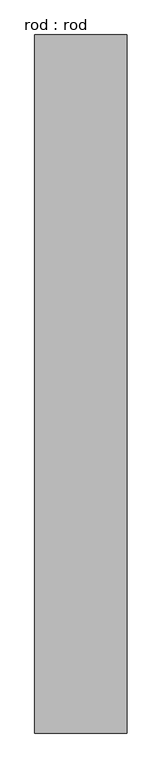
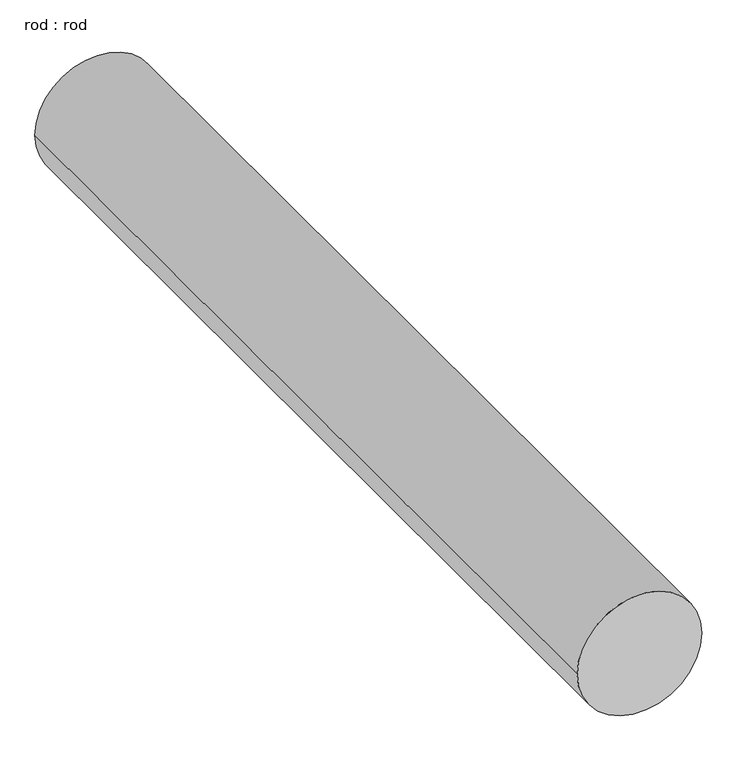
"""IFC4 building model written with IfcOpenShell, lengths in millimetres: proxy geometry, rod : rod."""

from ifc_helpers import new_model, si_unit, point, frame, frame_2d, origin, place, context, project, spatial, circle_curve, trimmed, segment, composite_curve, outline, extrude, source, transform, mapped, element, save


def rod_rod_aaba9445(model_context):
    return source(origin(), model_context, "Body", "SweptSolid", [
        extrude(outline(composite_curve([segment(trimmed(circle_curve(frame_2d((0.0108462, 0.0)), 200.0), [point((0.0108462, 200.0))], [point((0.0108462, -200.0))], False, "CARTESIAN"), True, "CONTINUOUS"), segment(trimmed(circle_curve(frame_2d((0.0108462, 0.0)), 200.0), [point((0.0108462, -200.0))], [point((0.0108462, 200.0))], False, "CARTESIAN"), True, "CONTINUOUS")], self_intersect=False)), frame((0.0, 2582.7286153, 0.0), z_axis=(0.0, 1.0, 0.0), x_axis=(0.0, 0.0, 1.0)), (0.0, 0.0, 1.0), 3020.0),
    ])


if __name__ == "__main__":
    model = new_model("IFC4")
    model_context = context("Model", 3, world=origin())
    ifc_project = project(units=[si_unit("LENGTHUNIT", "METRE", prefix="MILLI")], contexts=[model_context])
    site = spatial("IfcSite", under=ifc_project)
    building = spatial("IfcBuilding", under=site)
    placement = place(None, origin())
    rod_rod_shape = rod_rod_aaba9445(model_context)
    element("IfcBuildingElementProxy", 1, Name="rod : rod", ObjectType="rod : rod", at=placement, inside=building, context=model_context, shape_type="MappedRepresentation", body=[
        mapped(rod_rod_shape, transform((0.0, 0.0, 0.0), x_axis=(1.0, 0.0, 0.0), y_axis=(0.0, 1.0, 0.0), z_axis=(0.0, 0.0, 1.0))),
    ])
    save(model, "model.ifc")

# Revit data of these elements
# Type "rod : rod"
#   Default Elevation = 0
